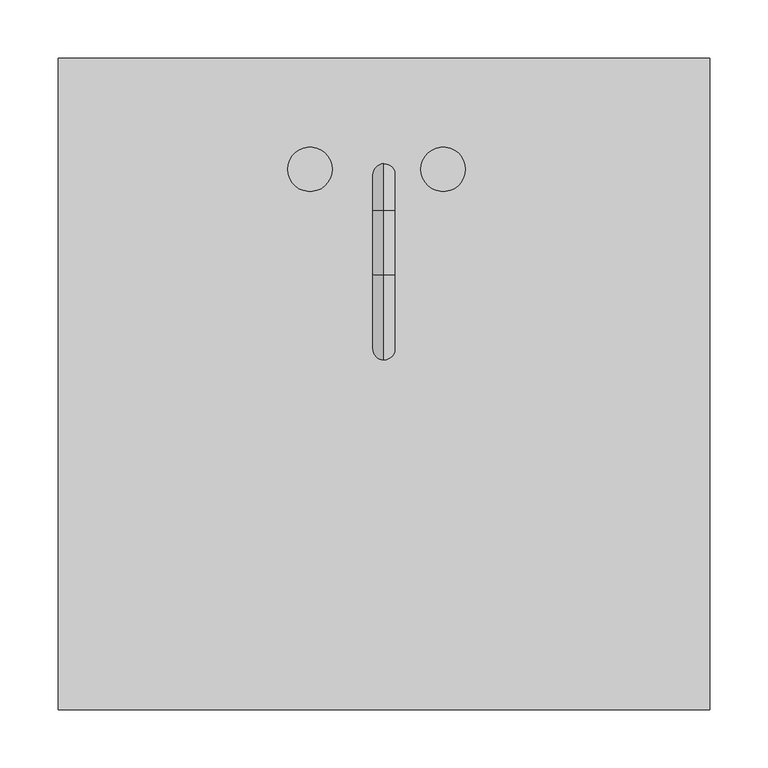
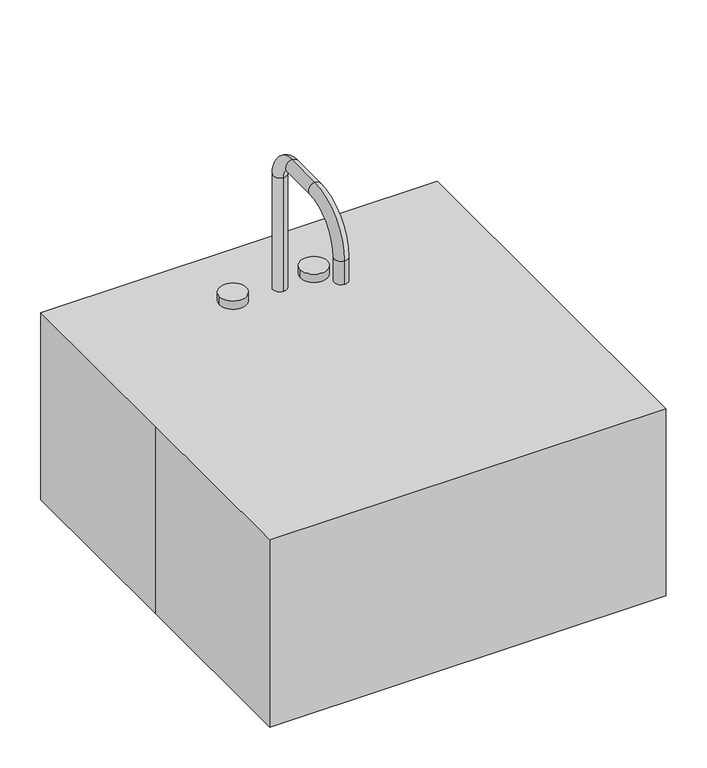
"""IFC4 building model written with IfcOpenShell, lengths in millimetres: proxy geometry, CS150 - Sink, SS, Single Compartment, 10x19x16 ID : CS150 - Sink, SS, Single Compartment, 10x19x16 ID."""

import ifcopenshell
import ifcopenshell.guid

model = None  # the IFC model being written
_history = None  # IfcOwnerHistory: only IFC2X3 demands one
_inside = {}  # id of a spatial element -> (the spatial element, [elements in it])
_under = {}  # id of a project, library or spatial element -> (it, [spatial elements below it])
_declared = {}  # id of a project -> (the project, [libraries it declares])
_typed = {}  # id of a type object -> (the type object, [elements of that type])
_made_of = {}  # id of a material, layer set ... -> (it, [elements and type objects made of it])


def new_model(schema):
    """Start an empty IFC model of exactly this schema.

    Asked for "IFC4X3", IfcOpenShell would pick the latest addendum, in which some entities
    have other attributes; the version numbers below select the first issue.
    IFC2X3 requires an IfcOwnerHistory on every rooted entity: one is made here for all.
    """
    global model, _history
    if schema == "IFC4X3":
        model = ifcopenshell.file(schema_version=(4, 3, 0, 0))
    else:
        model = ifcopenshell.file(schema=schema)
    _inside.clear()
    _under.clear()
    _declared.clear()
    _typed.clear()
    _made_of.clear()
    _history = None
    if model.schema == "IFC2X3":
        org = make("IfcOrganization", Name="unknown")
        user = make(
            "IfcPersonAndOrganization",
            ThePerson=make("IfcPerson", FamilyName="unknown"),
            TheOrganization=org,
        )
        app = make(
            "IfcApplication",
            ApplicationDeveloper=org,
            Version="unknown",
            ApplicationFullName="unknown",
            ApplicationIdentifier="unknown",
        )
        _history = make(
            "IfcOwnerHistory",
            OwningUser=user,
            OwningApplication=app,
            ChangeAction="ADDED",
            CreationDate=0,
        )
    return model


def make(cls, **values):
    """One entity of the class cls with the attributes given. An attribute that is None is left unset."""
    return model.create_entity(
        cls, **{name: value for name, value in values.items() if value is not None}
    )


def rooted(cls, **values):
    """An entity with a GlobalId (a new one), such as an element, a storey or a relation."""
    return make(cls, GlobalId=ifcopenshell.guid.new(), OwnerHistory=_history, **values)


def si_unit(unit_type, name, prefix=None):
    """IfcSIUnit, for example si_unit("LENGTHUNIT", "METRE", prefix="MILLI")."""
    return make("IfcSIUnit", UnitType=unit_type, Prefix=prefix, Name=name)


def assignment(units):
    """IfcUnitAssignment: the units of a project."""
    return None if units is None else make("IfcUnitAssignment", Units=units)


def point(xyz):
    """IfcCartesianPoint."""
    return None if xyz is None else make("IfcCartesianPoint", Coordinates=xyz)


def direction(xyz):
    """IfcDirection."""
    return None if xyz is None else make("IfcDirection", DirectionRatios=xyz)


def frame(location, z_axis=None, x_axis=None):
    """IfcAxis2Placement3D, a coordinate frame: its origin and axes. An axis left out is left unset."""
    return make(
        "IfcAxis2Placement3D",
        Location=point(location),
        Axis=direction(z_axis),
        RefDirection=direction(x_axis),
    )


def frame_2d(location, x_axis=None):
    """IfcAxis2Placement2D, a coordinate frame in the plane: its origin and x axis."""
    return make(
        "IfcAxis2Placement2D", Location=point(location), RefDirection=direction(x_axis)
    )


def origin():
    """The frame at (0, 0, 0) with its axes left unset."""
    return frame((0.0, 0.0, 0.0))


def origin_with_axes():
    """The frame at (0, 0, 0) with the z axis (0, 0, 1) and the x axis (1, 0, 0) written out."""
    return frame((0.0, 0.0, 0.0), z_axis=(0.0, 0.0, 1.0), x_axis=(1.0, 0.0, 0.0))


def origin_2d():
    """The frame at (0, 0) in the plane with its x axis left unset."""
    return frame_2d((0.0, 0.0))


def place(relative_to, where):
    """IfcLocalPlacement: puts the frame where relative to a parent placement (None: the world)."""
    return make(
        "IfcLocalPlacement", PlacementRelTo=relative_to, RelativePlacement=where
    )


def context(
    kind, dimensions, precision=None, world=None, true_north=None, identifier=None
):
    """IfcGeometricRepresentationContext, for example the 3D "Model" context."""
    return make(
        "IfcGeometricRepresentationContext",
        ContextIdentifier=identifier,
        ContextType=kind,
        CoordinateSpaceDimension=dimensions,
        Precision=precision,
        WorldCoordinateSystem=world,
        TrueNorth=true_north,
    )


def project(units=None, contexts=None):
    """IfcProject with its units and contexts."""
    return rooted(
        "IfcProject",
        Name="project",
        RepresentationContexts=contexts,
        UnitsInContext=assignment(units),
    )


def spatial(cls, under=None, at=None, **own):
    """A site, building, storey or space (cls), placed at a placement, below another one or the project."""
    s = rooted(cls, ObjectPlacement=at, **own)
    if under is not None:
        _under.setdefault(under.id(), (under, []))[1].append(s)
    return s


def polyline(points):
    """IfcPolyline through the points."""
    return make("IfcPolyline", Points=[point(p) for p in points])


def circle_curve(where, radius):
    """IfcCircle in the frame where."""
    return make("IfcCircle", Position=where, Radius=radius)


def ellipse_curve(where, semi_axis1, semi_axis2):
    """IfcEllipse in the frame where."""
    return make(
        "IfcEllipse", Position=where, SemiAxis1=semi_axis1, SemiAxis2=semi_axis2
    )


def trimmed(basis, trim1, trim2, sense, master):
    """IfcTrimmedCurve: the piece of a basis curve between two trims."""
    return make(
        "IfcTrimmedCurve",
        BasisCurve=basis,
        Trim1=trim1,
        Trim2=trim2,
        SenseAgreement=sense,
        MasterRepresentation=master,
    )


def segment(curve, same_sense, transition):
    """IfcCompositeCurveSegment."""
    return make(
        "IfcCompositeCurveSegment",
        Transition=transition,
        SameSense=same_sense,
        ParentCurve=curve,
    )


def composite_curve(segments, self_intersect=None):
    """IfcCompositeCurve: segments joined end to end."""
    return make("IfcCompositeCurve", Segments=segments, SelfIntersect=self_intersect)


def outline(outer, holes=None, kind="AREA"):
    """IfcArbitraryClosedProfileDef: a profile drawn as a closed curve; with holes, ...WithVoids."""
    if holes is None:
        return make("IfcArbitraryClosedProfileDef", ProfileType=kind, OuterCurve=outer)
    return make(
        "IfcArbitraryProfileDefWithVoids",
        ProfileType=kind,
        OuterCurve=outer,
        InnerCurves=holes,
    )


def extrude(swept, where, along, depth):
    """IfcExtrudedAreaSolid: the profile swept, set in the frame where, extruded along a direction by depth."""
    return make(
        "IfcExtrudedAreaSolid",
        SweptArea=swept,
        Position=where,
        ExtrudedDirection=direction(along),
        Depth=depth,
    )


def shape(context_of_items, identifier, shape_type, items):
    """IfcShapeRepresentation: the items that make up one representation, for example the "Body"."""
    return make(
        "IfcShapeRepresentation",
        ContextOfItems=context_of_items,
        RepresentationIdentifier=identifier,
        RepresentationType=shape_type,
        Items=items,
    )


def source(mapping_origin, context_of_items, identifier, shape_type, items):
    """IfcRepresentationMap: a shape defined once, which mapped items show again and again."""
    return make(
        "IfcRepresentationMap",
        MappingOrigin=mapping_origin,
        MappedRepresentation=shape(context_of_items, identifier, shape_type, items),
    )


def transform(
    local_origin,
    x_axis=None,
    y_axis=None,
    z_axis=None,
    scale=None,
    scale2=None,
    scale3=None,
    uniform=True,
):
    """IfcCartesianTransformationOperator3D, or its non-uniform kind. x_axis, y_axis, z_axis: its Axis1, 2, 3."""
    if uniform:
        return make(
            "IfcCartesianTransformationOperator3D",
            Axis1=direction(x_axis),
            Axis2=direction(y_axis),
            LocalOrigin=point(local_origin),
            Scale=scale,
            Axis3=direction(z_axis),
        )
    return make(
        "IfcCartesianTransformationOperator3DnonUniform",
        Axis1=direction(x_axis),
        Axis2=direction(y_axis),
        LocalOrigin=point(local_origin),
        Scale=scale,
        Axis3=direction(z_axis),
        Scale2=scale2,
        Scale3=scale3,
    )


def mapped(mapping_source, mapping_target):
    """IfcMappedItem: shows the shape of a source again, moved by a transform."""
    return make(
        "IfcMappedItem", MappingSource=mapping_source, MappingTarget=mapping_target
    )


def made_of(thing, what):
    """Note that an element or type object is made of a material, layer set ...; save() writes the relation."""
    if what is not None:
        _made_of.setdefault(what.id(), (what, []))[1].append(thing)
    return thing


def element(
    cls,
    number,
    at=None,
    inside=None,
    cuts=None,
    type_object=None,
    material=None,
    context=None,
    identifier="Body",
    shape_type=None,
    held_by="IfcProductDefinitionShape",
    body=None,
    shapes=None,
    **own,
):
    """One element of the class cls, such as IfcWall. Its Tag is "e" and its number.

    at: its placement. inside: the storey or other place that contains it. cuts: it is an
    opening in that element (IfcRelVoidsElement). A single representation is given by context,
    identifier, shape_type and body (its items); several are given by shapes. held_by: the class
    of the entity that holds the representations. save() writes the other relations.
    """
    e = rooted(cls, Tag="e%d" % number, ObjectPlacement=at, **own)
    if body is not None:
        shapes = [shape(context, identifier, shape_type, body)]
    if shapes is not None:
        e.Representation = make(held_by, Representations=shapes)
    if inside is not None:
        _inside.setdefault(inside.id(), (inside, []))[1].append(e)
    if cuts is not None:
        rooted(
            "IfcRelVoidsElement", RelatingBuildingElement=cuts, RelatedOpeningElement=e
        )
    if type_object is not None:
        _typed.setdefault(type_object.id(), (type_object, []))[1].append(e)
    return made_of(e, material)


def aggregate(whole, parts):
    """IfcRelAggregates: a whole, such as a stair, and the parts it consists of."""
    return rooted("IfcRelAggregates", RelatingObject=whole, RelatedObjects=parts)


def save(model, path):
    """Write the relations noted so far, then the file.

    IfcRelAggregates (storeys below a building ...), IfcRelContainedInSpatialStructure (elements
    in a storey), IfcRelDefinesByType, IfcRelAssociatesMaterial and IfcRelDeclares: one each for
    every whole, place, type object, material and project.
    """
    for whole, parts in _under.values():
        aggregate(whole, parts)
    for where, things in _inside.values():
        rooted(
            "IfcRelContainedInSpatialStructure",
            RelatedElements=things,
            RelatingStructure=where,
        )
    for kind, things in _typed.values():
        rooted("IfcRelDefinesByType", RelatedObjects=things, RelatingType=kind)
    for what, things in _made_of.values():
        rooted("IfcRelAssociatesMaterial", RelatedObjects=things, RelatingMaterial=what)
    for by, libraries in _declared.values():
        rooted("IfcRelDeclares", RelatingContext=by, RelatedDefinitions=libraries)
    model.write(path)


def plane_surface(at):
    """IfcPlane: the flat surface through the origin of the frame at, square to its z axis."""
    return make("IfcPlane", Position=at)


def cylinder_surface(at, radius):
    """IfcCylindricalSurface: all points at the distance radius from the z axis of the frame at."""
    return make("IfcCylindricalSurface", Position=at, Radius=radius)


def revolved_surface(curve, axis_point, axis_direction):
    """IfcSurfaceOfRevolution: the curve turned about the line through axis_point along axis_direction."""
    return make(
        "IfcSurfaceOfRevolution",
        SweptCurve=make("IfcArbitraryOpenProfileDef", ProfileType="CURVE", Curve=curve),
        AxisPosition=make("IfcAxis1Placement", Location=point(axis_point), Axis=direction(axis_direction)),
    )


def advanced_brep(points, edges, surfaces, faces):
    """IfcAdvancedBrep: a solid bounded by faces that lie on surfaces and meet in shared edges.

    An edge is (start, end): straight between two places in points (the first is 0);
    or (start, end, curve); or (start, end, curve, False) where it runs against its curve.
    A face is (place in surfaces, loops), or (place, loops, False) where it looks against
    its surface's normal. A loop lists edges by number (the first is 1), with a minus sign
    where the edge is run from its end to its start. The first loop is the outer one.
    """
    corners = [point(p) for p in points]
    vertices = [make("IfcVertexPoint", VertexGeometry=c) for c in corners]
    made = []
    for start, end, *more in edges:
        made.append(
            make(
                "IfcEdgeCurve",
                EdgeStart=vertices[start],
                EdgeEnd=vertices[end],
                EdgeGeometry=more[0] if more else make("IfcPolyline", Points=[corners[start], corners[end]]),
                SameSense=more[1] if len(more) > 1 else True,
            )
        )
    hull = []
    for where, loops, *sense in faces:
        bounds = []
        for j, loop in enumerate(loops):
            ring = [make("IfcOrientedEdge", EdgeElement=made[abs(k) - 1], Orientation=k > 0) for k in loop]
            bounds.append(
                make(
                    "IfcFaceOuterBound" if j == 0 else "IfcFaceBound",
                    Bound=make("IfcEdgeLoop", EdgeList=ring),
                    Orientation=True,
                )
            )
        hull.append(make("IfcAdvancedFace", Bounds=bounds, FaceSurface=surfaces[where], SameSense=sense[0] if sense else True))
    return make("IfcAdvancedBrep", Outer=make("IfcClosedShell", CfsFaces=hull))


def specialty_equipment_6fe3dbbb(model_context):
    return source(origin(), model_context, "Body", "SolidModel", [
        extrude(outline(composite_curve([segment(trimmed(circle_curve(frame_2d((139.6999999, 92.075)), 25.4), [point((139.6999999, 117.475))], [point((165.0999999, 92.075))], False, "CARTESIAN"), True, "CONTINUOUS"), segment(polyline([(165.0999999, 92.075), (165.0999999, -101.6)]), True, "CONTINUOUS"), segment(trimmed(circle_curve(frame_2d((139.6999999, -101.6)), 25.4), [point((165.0999999, -101.6))], [point((139.6999999, -127.0))], False, "CARTESIAN"), True, "CONTINUOUS"), segment(polyline([(139.6999999, -127.0), (-139.7000001, -127.0)]), True, "CONTINUOUS"), segment(trimmed(circle_curve(frame_2d((-139.7000001, -101.6)), 25.4), [point((-139.7000001, -127.0))], [point((-165.1000001, -101.6))], False, "CARTESIAN"), True, "CONTINUOUS"), segment(polyline([(-165.1000001, -101.6), (-165.1000001, 92.075)]), True, "CONTINUOUS"), segment(trimmed(circle_curve(frame_2d((-139.7000001, 92.075)), 25.4), [point((-165.1000001, 92.075))], [point((-139.7000001, 117.475))], False, "CARTESIAN"), True, "CONTINUOUS"), segment(polyline([(-139.7000001, 117.475), (139.6999999, 117.475)]), True, "CONTINUOUS")], self_intersect=False), holes=[composite_curve([segment(trimmed(circle_curve(origin_2d(), 12.7), [point((-12.7, 0.0))], [point((12.7, 0.0))], True, "CARTESIAN"), True, "CONTINUOUS"), segment(trimmed(circle_curve(origin_2d(), 12.7), [point((12.7, 0.0))], [point((-12.7, 0.0))], True, "CARTESIAN"), True, "CONTINUOUS")], self_intersect=False)]), origin_with_axes(), (0.0, 0.0, 1.0), 9.525),
        extrude(outline(polyline([(-279.4, 279.4), (279.4, 279.4), (279.4, -279.4), (-279.4, -279.4), (-279.4, 0.0), (-279.4, 279.4)])), origin_with_axes(), (0.0, 0.0, 1.0), 279.4),
        extrude(outline(composite_curve([segment(trimmed(circle_curve(frame_2d((76.1999999, 184.15)), 19.05), [point((76.1999999, 203.2))], [point((76.1999999, 165.1))], False, "CARTESIAN"), True, "CONTINUOUS"), segment(polyline([(76.1999999, 165.1), (-88.9000001, 165.1)]), True, "CONTINUOUS"), segment(trimmed(circle_curve(frame_2d((-88.9000001, 184.15)), 19.05), [point((-88.9000001, 165.1))], [point((-88.9000001, 203.2))], False, "CARTESIAN"), True, "CONTINUOUS"), segment(polyline([(-88.9000001, 203.2), (76.1999999, 203.2)]), True, "CONTINUOUS")], self_intersect=False), holes=[composite_curve([segment(trimmed(circle_curve(frame_2d((-1e-07, 179.3875)), 9.525), [point((-9.5250001, 179.3875))], [point((9.5249999, 179.3875))], True, "CARTESIAN"), True, "CONTINUOUS"), segment(trimmed(circle_curve(frame_2d((-1e-07, 179.3875)), 9.525), [point((9.5249999, 179.3875))], [point((-9.5250001, 179.3875))], True, "CARTESIAN"), True, "CONTINUOUS")], self_intersect=False)]), frame((0.0, 0.0, 228.6), z_axis=(0.0, 0.0, 1.0), x_axis=(1.0, 0.0, 0.0)), (0.0, 0.0, 1.0), 12.7),
        extrude(outline(composite_curve([segment(trimmed(circle_curve(frame_2d((-1e-07, 179.3875)), 12.7), [point((-12.7000001, 179.3875))], [point((12.6999999, 179.3875))], False, "CARTESIAN"), True, "CONTINUOUS"), segment(trimmed(circle_curve(frame_2d((-1e-07, 179.3875)), 12.7), [point((12.6999999, 179.3875))], [point((-12.7000001, 179.3875))], False, "CARTESIAN"), True, "CONTINUOUS")], self_intersect=False), holes=[composite_curve([segment(trimmed(circle_curve(frame_2d((-1e-07, 179.3875)), 9.525), [point((-9.5250001, 179.3875))], [point((9.5249999, 179.3875))], True, "CARTESIAN"), True, "CONTINUOUS"), segment(trimmed(circle_curve(frame_2d((-1e-07, 179.3875)), 9.525), [point((9.5249999, 179.3875))], [point((-9.5250001, 179.3875))], True, "CARTESIAN"), True, "CONTINUOUS")], self_intersect=False)]), frame((0.0, 0.0, 241.3), z_axis=(0.0, 0.0, 1.0), x_axis=(1.0, 0.0, 0.0)), (0.0, 0.0, 1.0), 12.7),
        advanced_brep(
        [(-1e-07, 188.9125, 228.6), (-1e-07, 169.8625, 228.6), (-1e-07, 188.9125, 449.2625), (-1e-07, 169.8625, 449.2625), (-1e-07, 149.225, 469.9), (-1e-07, 149.225, 488.95), (-1e-07, 93.6625, 488.95), (-1e-07, 93.6625, 469.9), (-1e-07, 39.6875, 415.925), (-1e-07, 20.6375, 415.925), (-1e-07, 20.6375, 381.0), (-1e-07, 39.6875, 381.0)],
        [
            (0, 1, circle_curve(frame((-1e-07, 179.3875, 228.6), z_axis=(0.0, 0.0, -1.0), x_axis=(0.0, -1.0, 0.0)), 9.525)),
            (1, 0, circle_curve(frame((-1e-07, 179.3875, 228.6), z_axis=(0.0, 0.0, -1.0), x_axis=(0.0, -1.0, 0.0)), 9.525)),
            (0, 2),
            (2, 3, circle_curve(frame((-1e-07, 179.3875, 449.2625), z_axis=(0.0, 0.0, -1.0), x_axis=(0.0, -1.0, 0.0)), 9.525)),
            (3, 1),
            (3, 2, circle_curve(frame((-1e-07, 179.3875, 449.2625), z_axis=(0.0, 0.0, -1.0), x_axis=(0.0, -1.0, 0.0)), 9.525)),
            (4, 3, circle_curve(frame((-1e-07, 149.225, 449.2625), z_axis=(-1.0, 0.0, 0.0), x_axis=(0.0, 1.0, 0.0)), 20.6375)),
            (2, 5, circle_curve(frame((-1e-07, 149.225, 449.2625), z_axis=(1.0, 0.0, 0.0), x_axis=(0.0, 1.0, 0.0)), 39.6875)),
            (5, 4, circle_curve(frame((-1e-07, 149.225, 479.425), z_axis=(0.0, 1.0, 0.0), x_axis=(0.0, 0.0, -1.0)), 9.525)),
            (4, 5, circle_curve(frame((-1e-07, 149.225, 479.425), z_axis=(0.0, 1.0, 0.0), x_axis=(0.0, 0.0, -1.0)), 9.525)),
            (5, 6),
            (6, 7, circle_curve(frame((-1e-07, 93.6625, 479.425), z_axis=(0.0, 1.0, 0.0), x_axis=(0.0, 0.0, -1.0)), 9.525)),
            (7, 4),
            (7, 6, circle_curve(frame((-1e-07, 93.6625, 479.425), z_axis=(0.0, 1.0, 0.0), x_axis=(0.0, 0.0, -1.0)), 9.525)),
            (8, 7, circle_curve(frame((-1e-07, 93.6625, 415.925), z_axis=(-1.0, 0.0, 0.0), x_axis=(0.0, 0.0, 1.0)), 53.975)),
            (6, 9, circle_curve(frame((-1e-07, 93.6625, 415.925), z_axis=(1.0, 0.0, 0.0), x_axis=(0.0, 0.0, 1.0)), 73.025)),
            (9, 8, circle_curve(frame((-1e-07, 30.1625, 415.925), z_axis=(0.0, 0.0, 1.0), x_axis=(0.0, 1.0, 0.0)), 9.525)),
            (8, 9, circle_curve(frame((-1e-07, 30.1625, 415.925), z_axis=(0.0, 0.0, 1.0), x_axis=(0.0, 1.0, 0.0)), 9.525)),
            (10, 11, circle_curve(frame((-1e-07, 30.1625, 381.0), z_axis=(0.0, 0.0, -1.0), x_axis=(0.0, 1.0, 0.0)), 9.525)),
            (11, 10, circle_curve(frame((-1e-07, 30.1625, 381.0), z_axis=(0.0, 0.0, -1.0), x_axis=(0.0, 1.0, 0.0)), 9.525)),
            (9, 10),
            (11, 8),
        ],
        [
            plane_surface(frame((-1e-07, 169.8625, 228.6), z_axis=(0.0, 0.0, -1.0), x_axis=(1.0, 0.0, 0.0))),
            cylinder_surface(frame((-1e-07, 179.3875, 228.6), z_axis=(0.0, 0.0, -1.0), x_axis=(0.0, -1.0, 0.0)), 9.525),
            revolved_surface(trimmed(ellipse_curve(frame((-1e-07, 179.3875, 449.2625), z_axis=(0.0, 0.0, -1.0), x_axis=(0.0, -1.0, 0.0)), 9.525, 9.525), [point((-1e-07, 188.9125, 449.2625))], [point((-1e-07, 169.8625, 449.2625))], True, "CARTESIAN"), (-1e-07, 149.225, 449.2625), (1.0, 0.0, 0.0)),
            revolved_surface(trimmed(ellipse_curve(frame((-1e-07, 179.3875, 449.2625), z_axis=(0.0, 0.0, -1.0), x_axis=(0.0, -1.0, 0.0)), 9.525, 9.525), [point((-1e-07, 169.8625, 449.2625))], [point((-1e-07, 188.9125, 449.2625))], True, "CARTESIAN"), (-1e-07, 149.225, 449.2625), (1.0, 0.0, 0.0)),
            cylinder_surface(frame((-1e-07, 149.225, 479.425), z_axis=(0.0, 1.0, 0.0), x_axis=(0.0, 0.0, -1.0)), 9.525),
            revolved_surface(trimmed(ellipse_curve(frame((-1e-07, 93.6625, 479.425), z_axis=(0.0, 1.0, 0.0), x_axis=(0.0, 0.0, -1.0)), 9.525, 9.525), [point((-1e-07, 93.6625, 488.95))], [point((-1e-07, 93.6625, 469.9))], True, "CARTESIAN"), (-1e-07, 93.6625, 415.925), (1.0, 0.0, 0.0)),
            revolved_surface(trimmed(ellipse_curve(frame((-1e-07, 93.6625, 479.425), z_axis=(0.0, 1.0, 0.0), x_axis=(0.0, 0.0, -1.0)), 9.525, 9.525), [point((-1e-07, 93.6625, 469.9))], [point((-1e-07, 93.6625, 488.95))], True, "CARTESIAN"), (-1e-07, 93.6625, 415.925), (1.0, 0.0, 0.0)),
            plane_surface(frame((-1e-07, 20.6375, 381.0), z_axis=(0.0, 0.0, -1.0), x_axis=(-1.0, 0.0, 0.0))),
            cylinder_surface(frame((-1e-07, 30.1625, 415.925), z_axis=(0.0, 0.0, 1.0), x_axis=(0.0, 1.0, 0.0)), 9.525),
        ],
        [
            (0, [[1, 2]]),
            (1, [[-1, 3, 4, 5]]),
            (1, [[-2, -5, 6, -3]]),
            (2, [[7, -4, 8, 9]]),
            (3, [[-8, -6, -7, 10]]),
            (4, [[-9, 11, 12, 13]]),
            (4, [[-10, -13, 14, -11]]),
            (5, [[15, -12, 16, 17]]),
            (6, [[-16, -14, -15, 18]]),
            (7, [[19, 20]]),
            (8, [[-17, 21, -20, 22]]),
            (8, [[-18, -22, -19, -21]]),
        ],
    ),
        extrude(outline(composite_curve([segment(trimmed(circle_curve(frame_2d((-63.5000001, 184.15)), 19.05), [point((-82.5500001, 184.15))], [point((-44.4500001, 184.15))], False, "CARTESIAN"), True, "CONTINUOUS"), segment(trimmed(circle_curve(frame_2d((-63.5000001, 184.15)), 19.05), [point((-44.4500001, 184.15))], [point((-82.5500001, 184.15))], False, "CARTESIAN"), True, "CONTINUOUS")], self_intersect=False)), frame((0.0, 0.0, 241.3), z_axis=(0.0, 0.0, 1.0), x_axis=(1.0, 0.0, 0.0)), (0.0, 0.0, 1.0), 50.8),
        extrude(outline(composite_curve([segment(trimmed(circle_curve(frame_2d((50.7999999, 184.15)), 19.05), [point((31.7499999, 184.15))], [point((69.8499999, 184.15))], False, "CARTESIAN"), True, "CONTINUOUS"), segment(trimmed(circle_curve(frame_2d((50.7999999, 184.15)), 19.05), [point((69.8499999, 184.15))], [point((31.7499999, 184.15))], False, "CARTESIAN"), True, "CONTINUOUS")], self_intersect=False)), frame((0.0, 0.0, 241.3), z_axis=(0.0, 0.0, 1.0), x_axis=(1.0, 0.0, 0.0)), (0.0, 0.0, 1.0), 50.8),
        advanced_brep(
        [(-139.7000001, 161.925, 0.0), (-139.7000001, 161.925, 215.9), (139.6999999, 161.925, 215.9), (139.6999999, 161.925, 0.0), (-139.7000001, 117.475, 0.0), (139.6999999, 117.475, 0.0), (-139.7000001, 117.475, 9.525), (139.6999999, 117.475, 9.525), (-139.7000001, 120.0634182, 9.525), (139.6999999, 120.0634182, 9.525), (-139.7000001, 139.0409272, 26.9146831), (139.6999999, 139.0409272, 26.9146831), (-139.7000001, 155.575, 215.9), (139.6999999, 155.575, 215.9), (209.5499999, 92.075, 0.0), (209.5499999, 92.075, 215.9), (165.0999999, 92.075, 0.0), (165.0999999, 92.075, 9.525), (167.6884181, 92.075, 9.525), (186.6659271, 92.075, 26.9146831), (203.1999999, 92.075, 215.9), (209.5499999, -101.6, 215.9), (209.5499999, -101.6, 0.0), (165.0999999, -101.6, 0.0), (165.0999999, -101.6, 9.525), (167.6884181, -101.6, 9.525), (186.6659271, -101.6, 26.9146831), (203.1999999, -101.6, 215.9), (139.6999999, -171.45, 0.0), (139.6999999, -171.45, 215.9), (139.6999999, -127.0, 0.0), (139.6999999, -127.0, 9.525), (139.6999999, -129.5884182, 9.525), (139.6999999, -148.5659272, 26.9146831), (139.6999999, -165.1, 215.9), (-139.7000001, -171.45, 215.9), (-139.7000001, -171.45, 0.0), (-139.7000001, -127.0, 0.0), (-139.7000001, -127.0, 9.525), (-139.7000001, -129.5884182, 9.525), (-139.7000001, -148.5659272, 26.9146831), (-139.7000001, -165.1, 215.9), (-209.5500001, -101.6, 0.0), (-209.5500001, -101.6, 215.9), (-165.1000001, -101.6, 0.0), (-165.1000001, -101.6, 9.525), (-167.6884183, -101.6, 9.525), (-186.6659273, -101.6, 26.9146831), (-203.2000001, -101.6, 215.9), (-209.5500001, 92.075, 215.9), (-209.5500001, 92.075, 0.0), (-165.1000001, 92.075, 0.0), (-165.1000001, 92.075, 9.525), (-167.6884183, 92.075, 9.525), (-186.6659273, 92.075, 26.9146831), (-203.2000001, 92.075, 215.9)],
        [
            (0, 1),
            (1, 2),
            (2, 3),
            (3, 0),
            (4, 0),
            (3, 5),
            (5, 4),
            (6, 4),
            (5, 7),
            (7, 6),
            (8, 6),
            (7, 9),
            (9, 8),
            (10, 8, circle_curve(frame((-139.7000001, 120.0634182, 28.575), z_axis=(-1.0, 0.0, 0.0), x_axis=(0.0, 1.0, 0.0)), 19.05)),
            (9, 11, circle_curve(frame((139.6999999, 120.0634182, 28.575), z_axis=(1.0, 0.0, 0.0), x_axis=(0.0, 1.0, 0.0)), 19.05)),
            (11, 10),
            (12, 10),
            (11, 13),
            (13, 12),
            (1, 12),
            (13, 2),
            (14, 3, circle_curve(frame((139.6999999, 92.075, 0.0), z_axis=(0.0, 0.0, 1.0), x_axis=(0.0, 1.0, 0.0)), 69.85)),
            (2, 15, circle_curve(frame((139.6999999, 92.075, 215.9), z_axis=(0.0, 0.0, -1.0), x_axis=(0.0, 1.0, 0.0)), 69.85)),
            (15, 14),
            (16, 5, circle_curve(frame((139.6999999, 92.075, 0.0), z_axis=(0.0, 0.0, 1.0), x_axis=(0.0, 1.0, 0.0)), 25.4)),
            (14, 16),
            (17, 7, circle_curve(frame((139.6999999, 92.075, 9.525), z_axis=(0.0, 0.0, 1.0), x_axis=(0.0, 1.0, 0.0)), 25.4)),
            (16, 17),
            (18, 9, circle_curve(frame((139.6999999, 92.075, 9.525), z_axis=(0.0, 0.0, 1.0), x_axis=(0.0, 1.0, 0.0)), 27.9884182)),
            (17, 18),
            (19, 11, circle_curve(frame((139.6999999, 92.075, 26.9146831), z_axis=(0.0, 0.0, 1.0), x_axis=(0.0, 1.0, 0.0)), 46.9659272)),
            (18, 19, circle_curve(frame((167.6884181, 92.075, 28.575), z_axis=(0.0, -1.0, 0.0), x_axis=(1.0, 0.0, 0.0)), 19.05)),
            (20, 13, circle_curve(frame((139.6999999, 92.075, 215.9), z_axis=(0.0, 0.0, 1.0), x_axis=(0.0, 1.0, 0.0)), 63.5)),
            (19, 20),
            (20, 15),
            (15, 21),
            (21, 22),
            (22, 14),
            (22, 23),
            (23, 16),
            (23, 24),
            (24, 17),
            (24, 25),
            (25, 18),
            (25, 26, circle_curve(frame((167.6884181, -101.6, 28.575), z_axis=(0.0, -1.0, 0.0), x_axis=(1.0, 0.0, 0.0)), 19.05)),
            (26, 19),
            (26, 27),
            (27, 20),
            (27, 21),
            (28, 22, circle_curve(frame((139.6999999, -101.6, 0.0), z_axis=(0.0, 0.0, 1.0), x_axis=(1.0, 0.0, 0.0)), 69.85)),
            (21, 29, circle_curve(frame((139.6999999, -101.6, 215.9), z_axis=(0.0, 0.0, -1.0), x_axis=(1.0, 0.0, 0.0)), 69.85)),
            (29, 28),
            (30, 23, circle_curve(frame((139.6999999, -101.6, 0.0), z_axis=(0.0, 0.0, 1.0), x_axis=(1.0, 0.0, 0.0)), 25.4)),
            (28, 30),
            (31, 24, circle_curve(frame((139.6999999, -101.6, 9.525), z_axis=(0.0, 0.0, 1.0), x_axis=(1.0, 0.0, 0.0)), 25.4)),
            (30, 31),
            (32, 25, circle_curve(frame((139.6999999, -101.6, 9.525), z_axis=(0.0, 0.0, 1.0), x_axis=(1.0, 0.0, 0.0)), 27.9884182)),
            (31, 32),
            (33, 26, circle_curve(frame((139.6999999, -101.6, 26.9146831), z_axis=(0.0, 0.0, 1.0), x_axis=(1.0, 0.0, 0.0)), 46.9659272)),
            (32, 33, circle_curve(frame((139.6999999, -129.5884182, 28.575), z_axis=(-1.0, 0.0, 0.0), x_axis=(0.0, -1.0, 0.0)), 19.05)),
            (34, 27, circle_curve(frame((139.6999999, -101.6, 215.9), z_axis=(0.0, 0.0, 1.0), x_axis=(1.0, 0.0, 0.0)), 63.5)),
            (33, 34),
            (34, 29),
            (29, 35),
            (35, 36),
            (36, 28),
            (36, 37),
            (37, 30),
            (37, 38),
            (38, 31),
            (38, 39),
            (39, 32),
            (39, 40, circle_curve(frame((-139.7000001, -129.5884182, 28.575), z_axis=(-1.0, 0.0, 0.0), x_axis=(0.0, -1.0, 0.0)), 19.05)),
            (40, 33),
            (40, 41),
            (41, 34),
            (41, 35),
            (42, 36, circle_curve(frame((-139.7000001, -101.6, 0.0), z_axis=(0.0, 0.0, 1.0), x_axis=(0.0, -1.0, 0.0)), 69.85)),
            (35, 43, circle_curve(frame((-139.7000001, -101.6, 215.9), z_axis=(0.0, 0.0, -1.0), x_axis=(0.0, -1.0, 0.0)), 69.85)),
            (43, 42),
            (44, 37, circle_curve(frame((-139.7000001, -101.6, 0.0), z_axis=(0.0, 0.0, 1.0), x_axis=(0.0, -1.0, 0.0)), 25.4)),
            (42, 44),
            (45, 38, circle_curve(frame((-139.7000001, -101.6, 9.525), z_axis=(0.0, 0.0, 1.0), x_axis=(0.0, -1.0, 0.0)), 25.4)),
            (44, 45),
            (46, 39, circle_curve(frame((-139.7000001, -101.6, 9.525), z_axis=(0.0, 0.0, 1.0), x_axis=(0.0, -1.0, 0.0)), 27.9884182)),
            (45, 46),
            (47, 40, circle_curve(frame((-139.7000001, -101.6, 26.9146831), z_axis=(0.0, 0.0, 1.0), x_axis=(0.0, -1.0, 0.0)), 46.9659272)),
            (46, 47, circle_curve(frame((-167.6884183, -101.6, 28.575), z_axis=(0.0, 1.0, 0.0), x_axis=(-1.0, 0.0, 0.0)), 19.05)),
            (48, 41, circle_curve(frame((-139.7000001, -101.6, 215.9), z_axis=(0.0, 0.0, 1.0), x_axis=(0.0, -1.0, 0.0)), 63.5)),
            (47, 48),
            (48, 43),
            (43, 49),
            (49, 50),
            (50, 42),
            (50, 51),
            (51, 44),
            (51, 52),
            (52, 45),
            (52, 53),
            (53, 46),
            (53, 54, circle_curve(frame((-167.6884183, 92.075, 28.575), z_axis=(0.0, 1.0, 0.0), x_axis=(-1.0, 0.0, 0.0)), 19.05)),
            (54, 47),
            (54, 55),
            (55, 48),
            (55, 49),
            (0, 50, circle_curve(frame((-139.7000001, 92.075, 0.0), z_axis=(0.0, 0.0, 1.0), x_axis=(-1.0, 0.0, 0.0)), 69.85)),
            (49, 1, circle_curve(frame((-139.7000001, 92.075, 215.9), z_axis=(0.0, 0.0, -1.0), x_axis=(-1.0, 0.0, 0.0)), 69.85)),
            (4, 51, circle_curve(frame((-139.7000001, 92.075, 0.0), z_axis=(0.0, 0.0, 1.0), x_axis=(-1.0, 0.0, 0.0)), 25.4)),
            (6, 52, circle_curve(frame((-139.7000001, 92.075, 9.525), z_axis=(0.0, 0.0, 1.0), x_axis=(-1.0, 0.0, 0.0)), 25.4)),
            (8, 53, circle_curve(frame((-139.7000001, 92.075, 9.525), z_axis=(0.0, 0.0, 1.0), x_axis=(-1.0, 0.0, 0.0)), 27.9884182)),
            (10, 54, circle_curve(frame((-139.7000001, 92.075, 26.9146831), z_axis=(0.0, 0.0, 1.0), x_axis=(-1.0, 0.0, 0.0)), 46.9659272)),
            (12, 55, circle_curve(frame((-139.7000001, 92.075, 215.9), z_axis=(0.0, 0.0, 1.0), x_axis=(-1.0, 0.0, 0.0)), 63.5)),
        ],
        [
            plane_surface(frame((-139.7000001, 161.925, 215.9), z_axis=(0.0, 1.0, 0.0), x_axis=(1.0, 0.0, 0.0))),
            plane_surface(frame((-139.7000001, 161.925, 0.0), z_axis=(0.0, 0.0, -1.0), x_axis=(1.0, 0.0, 0.0))),
            plane_surface(frame((-139.7000001, 117.475, 0.0), z_axis=(0.0, -1.0, 0.0), x_axis=(1.0, 0.0, 0.0))),
            plane_surface(frame((-139.7000001, 117.475, 9.525), z_axis=(0.0, 0.0, 1.0), x_axis=(1.0, 0.0, 0.0))),
            revolved_surface(polyline([(139.69999989999997, 139.1134182, 28.575), (-139.7000001, 139.1134182, 28.575)]), (-139.7000001, 120.0634182, 28.575), (1.0, 0.0, 0.0)),
            plane_surface(frame((-139.7000001, 139.0409272, 26.9146831), z_axis=(0.0, -0.9961946980917442, 0.08715574274767408), x_axis=(1.0, 0.0, 0.0))),
            plane_surface(frame((-139.7000001, 155.575, 215.9), z_axis=(0.0, 0.0, 1.0), x_axis=(1.0, 0.0, 0.0))),
            cylinder_surface(frame((139.6999999, 92.075, -647.7), z_axis=(0.0, 0.0, -1.0), x_axis=(0.0, 1.0, 0.0)), 69.85),
            plane_surface(frame((139.6999999, 92.075, 0.0), z_axis=(0.0, 0.0, -1.0), x_axis=(0.0, 1.0, 0.0))),
            revolved_surface(polyline([(139.6999999, 117.475, 0.0), (139.6999999, 117.475, 9.524999999999977)]), (139.6999999, 92.075, -647.7), (0.0, 0.0, -1.0)),
            plane_surface(frame((139.6999999, 92.075, 9.525), z_axis=(0.0, 0.0, 1.0), x_axis=(0.0, 1.0, 0.0))),
            revolved_surface(trimmed(ellipse_curve(frame((139.6999999, 120.0634182, 28.575), z_axis=(1.0, 0.0, 0.0), x_axis=(0.0, 1.0, 0.0)), 19.05, 19.05), [point((139.6999999, 120.0634182, 9.525))], [point((139.6999999, 139.0409272, 26.9146831))], True, "CARTESIAN"), (139.6999999, 92.075, -647.7), (0.0, 0.0, -1.0)),
            revolved_surface(polyline([(139.6999999, 139.0409272, 26.9146831), (139.6999999, 155.575, 215.9)]), (139.6999999, 92.075, -647.7), (0.0, 0.0, -1.0)),
            plane_surface(frame((139.6999999, 92.075, 215.9), z_axis=(0.0, 0.0, 1.0), x_axis=(0.0, 1.0, 0.0))),
            plane_surface(frame((209.5499999, 92.075, 215.9), z_axis=(1.0, 0.0, 0.0), x_axis=(0.0, -1.0, 0.0))),
            plane_surface(frame((209.5499999, 92.075, 0.0), z_axis=(0.0, 0.0, -1.0), x_axis=(0.0, -1.0, 0.0))),
            plane_surface(frame((165.0999999, 92.075, 0.0), z_axis=(-1.0, 0.0, 0.0), x_axis=(0.0, -1.0, 0.0))),
            plane_surface(frame((165.0999999, 92.075, 9.525), z_axis=(0.0, 0.0, 1.0), x_axis=(0.0, -1.0, 0.0))),
            revolved_surface(polyline([(186.73841810000002, -101.60000000000001, 28.575), (186.73841810000002, 92.075, 28.575)]), (167.6884181, 92.075, 28.575), (0.0, -1.0, 0.0)),
            plane_surface(frame((186.6659271, 92.075, 26.9146831), z_axis=(-0.9961946980917442, 0.0, 0.08715574274767408), x_axis=(0.0, -1.0, 0.0))),
            plane_surface(frame((203.1999999, 92.075, 215.9), z_axis=(0.0, 0.0, 1.0), x_axis=(0.0, -1.0, 0.0))),
            cylinder_surface(frame((139.6999999, -101.6, -647.7), z_axis=(0.0, 0.0, -1.0), x_axis=(1.0, 0.0, 0.0)), 69.85),
            plane_surface(frame((139.6999999, -101.6, 0.0), z_axis=(0.0, 0.0, -1.0), x_axis=(1.0, 0.0, 0.0))),
            revolved_surface(polyline([(165.0999999, -101.6, 0.0), (165.0999999, -101.6, 9.524999999999977)]), (139.6999999, -101.6, -647.7), (0.0, 0.0, -1.0)),
            plane_surface(frame((139.6999999, -101.6, 9.525), z_axis=(0.0, 0.0, 1.0), x_axis=(1.0, 0.0, 0.0))),
            revolved_surface(trimmed(ellipse_curve(frame((167.6884181, -101.6, 28.575), z_axis=(0.0, -1.0, 0.0), x_axis=(1.0, 0.0, 0.0)), 19.05, 19.05), [point((167.6884181, -101.6, 9.525))], [point((186.6659271, -101.6, 26.9146831))], True, "CARTESIAN"), (139.6999999, -101.6, -647.7), (0.0, 0.0, -1.0)),
            revolved_surface(polyline([(186.6659271, -101.6, 26.9146831), (203.1999999, -101.6, 215.9)]), (139.6999999, -101.6, -647.7), (0.0, 0.0, -1.0)),
            plane_surface(frame((139.6999999, -101.6, 215.9), z_axis=(0.0, 0.0, 1.0), x_axis=(1.0, 0.0, 0.0))),
            plane_surface(frame((139.6999999, -171.45, 215.9), z_axis=(0.0, -1.0, 0.0), x_axis=(-1.0, 0.0, 0.0))),
            plane_surface(frame((139.6999999, -171.45, 0.0), z_axis=(0.0, 0.0, -1.0), x_axis=(-1.0, 0.0, 0.0))),
            plane_surface(frame((139.6999999, -127.0, 0.0), z_axis=(0.0, 1.0, 0.0), x_axis=(-1.0, 0.0, 0.0))),
            plane_surface(frame((139.6999999, -127.0, 9.525), z_axis=(0.0, 0.0, 1.0), x_axis=(-1.0, 0.0, 0.0))),
            revolved_surface(polyline([(-139.70000009999998, -148.63841820000002, 28.575), (139.6999999, -148.63841820000002, 28.575)]), (139.6999999, -129.5884182, 28.575), (-1.0, 0.0, 0.0)),
            plane_surface(frame((139.6999999, -148.5659272, 26.9146831), z_axis=(0.0, 0.9961946980917442, 0.08715574274767408), x_axis=(-1.0, 0.0, 0.0))),
            plane_surface(frame((139.6999999, -165.1, 215.9), z_axis=(0.0, 0.0, 1.0), x_axis=(-1.0, 0.0, 0.0))),
            cylinder_surface(frame((-139.7000001, -101.6, -647.7), z_axis=(0.0, 0.0, -1.0), x_axis=(0.0, -1.0, 0.0)), 69.85),
            plane_surface(frame((-139.7000001, -101.6, 0.0), z_axis=(0.0, 0.0, -1.0), x_axis=(0.0, -1.0, 0.0))),
            revolved_surface(polyline([(-139.7000001, -127.0, 0.0), (-139.7000001, -127.0, 9.524999999999977)]), (-139.7000001, -101.6, -647.7), (0.0, 0.0, -1.0)),
            plane_surface(frame((-139.7000001, -101.6, 9.525), z_axis=(0.0, 0.0, 1.0), x_axis=(0.0, -1.0, 0.0))),
            revolved_surface(trimmed(ellipse_curve(frame((-139.7000001, -129.5884182, 28.575), z_axis=(-1.0, 0.0, 0.0), x_axis=(0.0, -1.0, 0.0)), 19.05, 19.05), [point((-139.7000001, -129.5884182, 9.525))], [point((-139.7000001, -148.5659272, 26.9146831))], True, "CARTESIAN"), (-139.7000001, -101.6, -647.7), (0.0, 0.0, -1.0)),
            revolved_surface(polyline([(-139.7000001, -148.5659272, 26.9146831), (-139.7000001, -165.1, 215.9)]), (-139.7000001, -101.6, -647.7), (0.0, 0.0, -1.0)),
            plane_surface(frame((-139.7000001, -101.6, 215.9), z_axis=(0.0, 0.0, 1.0), x_axis=(0.0, -1.0, 0.0))),
            plane_surface(frame((-209.5500001, -101.6, 215.9), z_axis=(-1.0, 0.0, 0.0), x_axis=(0.0, 1.0, 0.0))),
            plane_surface(frame((-209.5500001, -101.6, 0.0), z_axis=(0.0, 0.0, -1.0), x_axis=(0.0, 1.0, 0.0))),
            plane_surface(frame((-165.1000001, -101.6, 0.0), z_axis=(1.0, 0.0, 0.0), x_axis=(0.0, 1.0, 0.0))),
            plane_surface(frame((-165.1000001, -101.6, 9.525), z_axis=(0.0, 0.0, 1.0), x_axis=(0.0, 1.0, 0.0))),
            revolved_surface(polyline([(-186.7384183, 92.07500000000002, 28.575), (-186.7384183, -101.6, 28.575)]), (-167.6884183, -101.6, 28.575), (0.0, 1.0, 0.0)),
            plane_surface(frame((-186.6659273, -101.6, 26.9146831), z_axis=(0.9961946980917442, 0.0, 0.08715574274767408), x_axis=(0.0, 1.0, 0.0))),
            plane_surface(frame((-203.2000001, -101.6, 215.9), z_axis=(0.0, 0.0, 1.0), x_axis=(0.0, 1.0, 0.0))),
            cylinder_surface(frame((-139.7000001, 92.075, -647.7), z_axis=(0.0, 0.0, -1.0), x_axis=(-1.0, 0.0, 0.0)), 69.85),
            plane_surface(frame((-139.7000001, 92.075, 0.0), z_axis=(0.0, 0.0, -1.0), x_axis=(-1.0, 0.0, 0.0))),
            revolved_surface(polyline([(-165.10000010000002, 92.075, 0.0), (-165.10000010000002, 92.075, 9.524999999999977)]), (-139.7000001, 92.075, -647.7), (0.0, 0.0, -1.0)),
            plane_surface(frame((-139.7000001, 92.075, 9.525), z_axis=(0.0, 0.0, 1.0), x_axis=(-1.0, 0.0, 0.0))),
            revolved_surface(trimmed(ellipse_curve(frame((-167.6884183, 92.075, 28.575), z_axis=(0.0, 1.0, 0.0), x_axis=(-1.0, 0.0, 0.0)), 19.05, 19.05), [point((-167.6884183, 92.075, 9.525))], [point((-186.6659273, 92.075, 26.9146831))], True, "CARTESIAN"), (-139.7000001, 92.075, -647.7), (0.0, 0.0, -1.0)),
            revolved_surface(polyline([(-186.6659273, 92.075, 26.9146831), (-203.2000001, 92.075, 215.9)]), (-139.7000001, 92.075, -647.7), (0.0, 0.0, -1.0)),
            plane_surface(frame((-139.7000001, 92.075, 215.9), z_axis=(0.0, 0.0, 1.0), x_axis=(-1.0, 0.0, 0.0))),
        ],
        [
            (0, [[1, 2, 3, 4]]),
            (1, [[5, -4, 6, 7]]),
            (2, [[8, -7, 9, 10]]),
            (3, [[11, -10, 12, 13]]),
            (4, [[14, -13, 15, 16]]),
            (5, [[17, -16, 18, 19]]),
            (6, [[20, -19, 21, -2]]),
            (7, [[22, -3, 23, 24]]),
            (8, [[25, -6, -22, 26]]),
            (9, [[27, -9, -25, 28]]),
            (10, [[29, -12, -27, 30]]),
            (11, [[31, -15, -29, 32]]),
            (12, [[33, -18, -31, 34]]),
            (13, [[-23, -21, -33, 35]]),
            (14, [[-24, 36, 37, 38]]),
            (15, [[-26, -38, 39, 40]]),
            (16, [[-28, -40, 41, 42]]),
            (17, [[-30, -42, 43, 44]]),
            (18, [[-32, -44, 45, 46]]),
            (19, [[-34, -46, 47, 48]]),
            (20, [[-35, -48, 49, -36]]),
            (21, [[50, -37, 51, 52]]),
            (22, [[53, -39, -50, 54]]),
            (23, [[55, -41, -53, 56]]),
            (24, [[57, -43, -55, 58]]),
            (25, [[59, -45, -57, 60]]),
            (26, [[61, -47, -59, 62]]),
            (27, [[-51, -49, -61, 63]]),
            (28, [[-52, 64, 65, 66]]),
            (29, [[-54, -66, 67, 68]]),
            (30, [[-56, -68, 69, 70]]),
            (31, [[-58, -70, 71, 72]]),
            (32, [[-60, -72, 73, 74]]),
            (33, [[-62, -74, 75, 76]]),
            (34, [[-63, -76, 77, -64]]),
            (35, [[78, -65, 79, 80]]),
            (36, [[81, -67, -78, 82]]),
            (37, [[83, -69, -81, 84]]),
            (38, [[85, -71, -83, 86]]),
            (39, [[87, -73, -85, 88]]),
            (40, [[89, -75, -87, 90]]),
            (41, [[-79, -77, -89, 91]]),
            (42, [[-80, 92, 93, 94]]),
            (43, [[-82, -94, 95, 96]]),
            (44, [[-84, -96, 97, 98]]),
            (45, [[-86, -98, 99, 100]]),
            (46, [[-88, -100, 101, 102]]),
            (47, [[-90, -102, 103, 104]]),
            (48, [[-91, -104, 105, -92]]),
            (49, [[106, -93, 107, -1]]),
            (50, [[108, -95, -106, -5]]),
            (51, [[109, -97, -108, -8]]),
            (52, [[110, -99, -109, -11]]),
            (53, [[111, -101, -110, -14]]),
            (54, [[112, -103, -111, -17]]),
            (55, [[-107, -105, -112, -20]]),
        ],
    ),
        extrude(outline(composite_curve([segment(trimmed(circle_curve(frame_2d((-177.8, -139.7)), 63.5), [point((-177.8, -203.2))], [point((-241.3, -139.7))], False, "CARTESIAN"), True, "CONTINUOUS"), segment(polyline([(-241.3, -139.7), (-241.3, 139.7)]), True, "CONTINUOUS"), segment(trimmed(circle_curve(frame_2d((-177.8, 139.7)), 63.5), [point((-241.3, 139.7))], [point((-177.8, 203.2))], False, "CARTESIAN"), True, "CONTINUOUS"), segment(polyline([(-177.8, 203.2), (177.7999999, 203.2)]), True, "CONTINUOUS"), segment(trimmed(circle_curve(frame_2d((177.7999999, 139.7)), 63.5), [point((177.7999999, 203.2))], [point((241.2999999, 139.7))], False, "CARTESIAN"), True, "CONTINUOUS"), segment(polyline([(241.2999999, 139.7), (241.2999999, -139.7)]), True, "CONTINUOUS"), segment(trimmed(circle_curve(frame_2d((177.7999999, -139.7)), 63.5), [point((241.2999999, -139.7))], [point((177.7999999, -203.2))], False, "CARTESIAN"), True, "CONTINUOUS"), segment(polyline([(177.7999999, -203.2), (-177.8, -203.2)]), True, "CONTINUOUS")], self_intersect=False), holes=[composite_curve([segment(polyline([(139.6999999, 155.575), (-139.7000001, 155.575)]), True, "CONTINUOUS"), segment(trimmed(circle_curve(frame_2d((-139.7000001, 92.075)), 63.5), [point((-139.7000001, 155.575))], [point((-203.2000001, 92.075))], True, "CARTESIAN"), True, "CONTINUOUS"), segment(polyline([(-203.2000001, 92.075), (-203.2000001, -101.6)]), True, "CONTINUOUS"), segment(trimmed(circle_curve(frame_2d((-139.7000001, -101.6)), 63.5), [point((-203.2000001, -101.6))], [point((-139.7000001, -165.1))], True, "CARTESIAN"), True, "CONTINUOUS"), segment(polyline([(-139.7000001, -165.1), (139.6999999, -165.1)]), True, "CONTINUOUS"), segment(trimmed(circle_curve(frame_2d((139.6999999, -101.6)), 63.5), [point((139.6999999, -165.1))], [point((203.1999999, -101.6))], True, "CARTESIAN"), True, "CONTINUOUS"), segment(polyline([(203.1999999, -101.6), (203.1999999, 92.075)]), True, "CONTINUOUS"), segment(trimmed(circle_curve(frame_2d((139.6999999, 92.075)), 63.5), [point((203.1999999, 92.075))], [point((139.6999999, 155.575))], True, "CARTESIAN"), True, "CONTINUOUS")], self_intersect=False)]), frame((0.0, 0.0, 215.9), z_axis=(0.0, 0.0, 1.0), x_axis=(1.0, 0.0, 0.0)), (0.0, 0.0, 1.0), 12.7),
    ])


if __name__ == "__main__":
    model = new_model("IFC4")
    model_context = context("Model", 3, world=origin())
    ifc_project = project(units=[si_unit("LENGTHUNIT", "METRE", prefix="MILLI")], contexts=[model_context])
    site = spatial("IfcSite", under=ifc_project)
    building = spatial("IfcBuilding", under=site)
    placement = place(None, origin())
    specialty_equipment_shape = specialty_equipment_6fe3dbbb(model_context)
    element("IfcBuildingElementProxy", 1, Name="CS150 - Sink, SS, Single Compartment, 10x19x16 ID : CS150 - Sink, SS, Single Compartment, 10x19x16 ID", ObjectType="CS150 - Sink, SS, Single Compartment, 10x19x16 ID : CS150 - Sink, SS, Single Compartment, 10x19x16 ID", at=placement, inside=building, context=model_context, shape_type="MappedRepresentation", body=[
        mapped(specialty_equipment_shape, transform((0.0, 0.0, 0.0), x_axis=(1.0, 0.0, 0.0), y_axis=(0.0, 1.0, 0.0), z_axis=(0.0, 0.0, 1.0))),
    ])
    save(model, "model.ifc")

# Revit data of these elements
# Type "CS150 - Sink, SS, Single Compartment, 10x19x16 ID : CS150 - Sink, SS, Single Compartment, 10x19x16 ID"
#   Watts2 = "0"
#   Watts1 = "0"
#   Unit_Issue = "EA"
#   UTIL_6_Misc = "-"
#   UTIL_5_NonMedGas = "-"
#   UTIL_4_MiscGas = "-"
#   UTIL_3_MedGas = "-"
#   UTIL_2_Elec = "-"
#   UTIL_1_WaterDrain = "D"
#   Nomenclature = "Sink, SS, Single Compartment, 10x19x16 ID"
#   NSN = "6530"
#   Location [instance default] = ""
#   JSN = "CS150"
#   Fund_Source_VA = "-"
#   Fund_Source_Navy = "-"
#   Fund_Source_Army = "-"
#   Fund_Source_AF = "-"
#   ELEC_Volts2 = "0"
#   ELEC_Volts1 = "0"
#   ELEC_Phase2 = "0"
#   ELEC_Phase1 = "0"
#   ELEC_HertzSwitch = "0"
#   ELEC_HertzDependent = "0"
#   ELEC_Hertz = "0"
#   ELEC_Amps2 = "0"
#   ELEC_Amps1 = "0"
#   DetailDescription = "Single compartment stainless steel sink, drop-in, self-rimming, ledge-type, connected with a drain and provided with a mixing faucet. It shall also be provided with pre-punched fixture holes on 4\" center, integral back ledge to accommodate deck-mounted fixtures, brushed/polished interior and top surfaces, and sound deadened. Recommended for use in suspended or U/C/B sink cabinets having a high plastic laminate or Chemsurf laminate countertop/work surface. Coordinate actual outside sink dimensions with the actual clear dimension of cabinet specified to ensure that they are compatible. For general purpose use throughout the facility."
#   CAT_VA = "A"
#   CAT_Navy = "A"
#   CAT_IHS = "-"
#   CAT_Army = "A"
#   CAT_AF = "A"
#   BTUperhour = "0"
#   Weight_IP = 32
#   DIM_Width_IP = 1' - 10"
#   DIM_Height_IP = 0' - 11"
#   DIM_Depth_IP = 1' - 10"
#   Faucet Material = Metal - Steel, Polished
#   Basin Material = Default
#   Assembly Code = ""
# Element 1 (IfcBuildingElementProxy, "CS150 - Sink, SS, Single Compartment, 10x19x16 ID : CS150 - Sink, SS, Single Compartment, 10x19x16 ID")
#   Location = "TRPE1"
#   Materials on its faces: "Default", "Metal - Steel, Polished", "EquipSpace"
# Materials
#   "Metal - Steel, Polished": class "Unassigned", colour RGB 57 57 57, transparency 0
#   "Default": class "Miscellaneous", colour RGB 127 127 127, transparency 0
#   "EquipSpace": class "Unassigned", colour RGB 221 217 195, transparency 0.5
